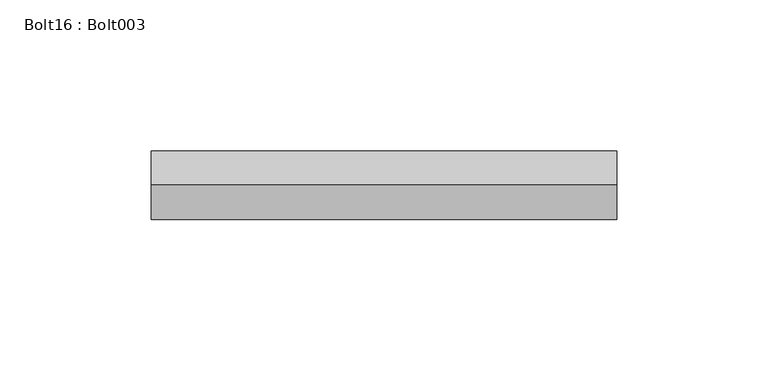
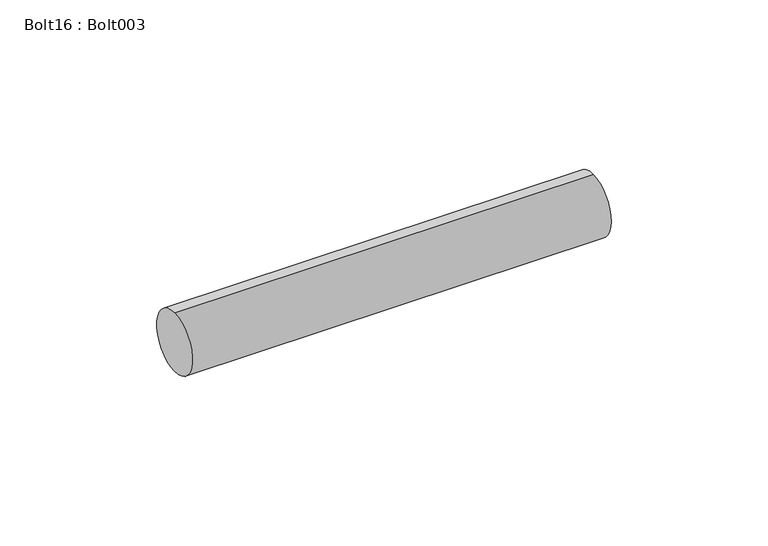
"""IFC4 building model written with IfcOpenShell, lengths in millimetres: proxy geometry, Bolt16 : Bolt003."""

from ifc_helpers import new_model, si_unit, point, frame, frame_2d, origin, place, context, project, spatial, circle_curve, trimmed, segment, composite_curve, outline, extrude, source, transform, mapped, element, save


def bolt16_bolt003_f80aea55(model_context):
    return source(origin(), model_context, "Body", "SweptSolid", [
        extrude(outline(composite_curve([segment(trimmed(circle_curve(frame_2d((1896.5882072, 39910.0063132)), 11.4045168), [point((1896.5882072, 39921.41083))], [point((1896.5882072, 39898.6017964))], False, "CARTESIAN"), True, "CONTINUOUS"), segment(trimmed(circle_curve(frame_2d((1896.5882072, 39910.0063132)), 11.4045168), [point((1896.5882072, 39898.6017964))], [point((1896.5882072, 39921.41083))], False, "CARTESIAN"), True, "CONTINUOUS")], self_intersect=False)), frame((10287.3140827, 0.0, 0.0), z_axis=(1.0, 0.0, 0.0), x_axis=(0.0, 1.0, 0.0)), (0.0, 0.0, 1.0), 154.0602393),
    ])


if __name__ == "__main__":
    model = new_model("IFC4")
    model_context = context("Model", 3, world=origin())
    ifc_project = project(units=[si_unit("LENGTHUNIT", "METRE", prefix="MILLI")], contexts=[model_context])
    site = spatial("IfcSite", under=ifc_project)
    building = spatial("IfcBuilding", under=site)
    placement = place(None, origin())
    bolt16_bolt003_shape = bolt16_bolt003_f80aea55(model_context)
    element("IfcBuildingElementProxy", 1, Name="Bolt16 : Bolt003", ObjectType="Bolt16 : Bolt003", at=placement, inside=building, context=model_context, shape_type="MappedRepresentation", body=[
        mapped(bolt16_bolt003_shape, transform((0.0, 0.0, 0.0), x_axis=(1.0, 0.0, 0.0), y_axis=(0.0, 1.0, 0.0), z_axis=(0.0, 0.0, 1.0))),
    ])
    save(model, "model.ifc")

# Revit data of these elements
# Type "Bolt16 : Bolt003"
#   NameOverride = "Bolt003"
# Element 1 (IfcBuildingElementProxy, "Bolt16 : Bolt003")
#   Materials on its faces: "TUBE STEEL STRINGER WELDED TO ANCHORED STEEL PLATE - SEE STRUCT DWGS"
# Materials
#   "TUBE STEEL STRINGER WELDED TO ANCHORED STEEL PLATE - SEE STRUCT DWGS": class "Unassigned", colour RGB 128 128 128, transparency 0, Cost = 0
